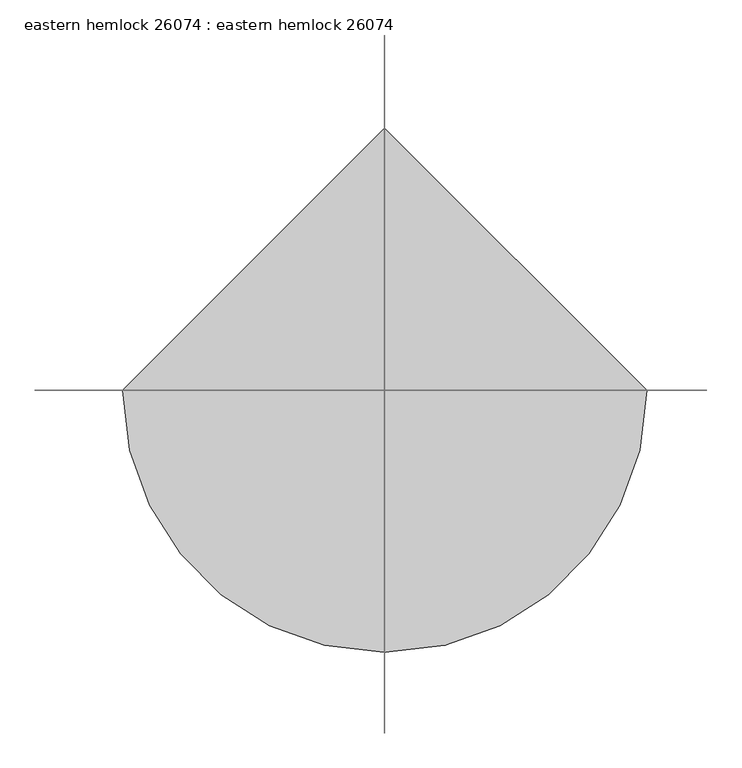
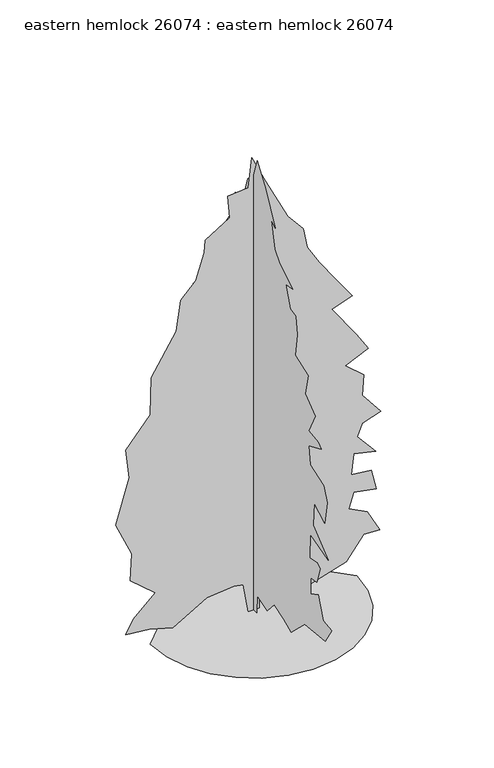
"""IFC4 building model written with IfcOpenShell, lengths in millimetres: proxy geometry, eastern hemlock 26074 : eastern hemlock 26074."""

import ifcopenshell
import ifcopenshell.guid

model = None  # the IFC model being written
_history = None  # IfcOwnerHistory: only IFC2X3 demands one
_inside = {}  # id of a spatial element -> (the spatial element, [elements in it])
_under = {}  # id of a project, library or spatial element -> (it, [spatial elements below it])
_declared = {}  # id of a project -> (the project, [libraries it declares])
_typed = {}  # id of a type object -> (the type object, [elements of that type])
_made_of = {}  # id of a material, layer set ... -> (it, [elements and type objects made of it])


def new_model(schema):
    """Start an empty IFC model of exactly this schema.

    Asked for "IFC4X3", IfcOpenShell would pick the latest addendum, in which some entities
    have other attributes; the version numbers below select the first issue.
    IFC2X3 requires an IfcOwnerHistory on every rooted entity: one is made here for all.
    """
    global model, _history
    if schema == "IFC4X3":
        model = ifcopenshell.file(schema_version=(4, 3, 0, 0))
    else:
        model = ifcopenshell.file(schema=schema)
    _inside.clear()
    _under.clear()
    _declared.clear()
    _typed.clear()
    _made_of.clear()
    _history = None
    if model.schema == "IFC2X3":
        org = make("IfcOrganization", Name="unknown")
        user = make(
            "IfcPersonAndOrganization",
            ThePerson=make("IfcPerson", FamilyName="unknown"),
            TheOrganization=org,
        )
        app = make(
            "IfcApplication",
            ApplicationDeveloper=org,
            Version="unknown",
            ApplicationFullName="unknown",
            ApplicationIdentifier="unknown",
        )
        _history = make(
            "IfcOwnerHistory",
            OwningUser=user,
            OwningApplication=app,
            ChangeAction="ADDED",
            CreationDate=0,
        )
    return model


def make(cls, **values):
    """One entity of the class cls with the attributes given. An attribute that is None is left unset."""
    return model.create_entity(
        cls, **{name: value for name, value in values.items() if value is not None}
    )


def rooted(cls, **values):
    """An entity with a GlobalId (a new one), such as an element, a storey or a relation."""
    return make(cls, GlobalId=ifcopenshell.guid.new(), OwnerHistory=_history, **values)


def si_unit(unit_type, name, prefix=None):
    """IfcSIUnit, for example si_unit("LENGTHUNIT", "METRE", prefix="MILLI")."""
    return make("IfcSIUnit", UnitType=unit_type, Prefix=prefix, Name=name)


def assignment(units):
    """IfcUnitAssignment: the units of a project."""
    return None if units is None else make("IfcUnitAssignment", Units=units)


def point(xyz):
    """IfcCartesianPoint."""
    return None if xyz is None else make("IfcCartesianPoint", Coordinates=xyz)


def direction(xyz):
    """IfcDirection."""
    return None if xyz is None else make("IfcDirection", DirectionRatios=xyz)


def frame(location, z_axis=None, x_axis=None):
    """IfcAxis2Placement3D, a coordinate frame: its origin and axes. An axis left out is left unset."""
    return make(
        "IfcAxis2Placement3D",
        Location=point(location),
        Axis=direction(z_axis),
        RefDirection=direction(x_axis),
    )


def origin():
    """The frame at (0, 0, 0) with its axes left unset."""
    return frame((0.0, 0.0, 0.0))


def place(relative_to, where):
    """IfcLocalPlacement: puts the frame where relative to a parent placement (None: the world)."""
    return make(
        "IfcLocalPlacement", PlacementRelTo=relative_to, RelativePlacement=where
    )


def context(
    kind, dimensions, precision=None, world=None, true_north=None, identifier=None
):
    """IfcGeometricRepresentationContext, for example the 3D "Model" context."""
    return make(
        "IfcGeometricRepresentationContext",
        ContextIdentifier=identifier,
        ContextType=kind,
        CoordinateSpaceDimension=dimensions,
        Precision=precision,
        WorldCoordinateSystem=world,
        TrueNorth=true_north,
    )


def project(units=None, contexts=None):
    """IfcProject with its units and contexts."""
    return rooted(
        "IfcProject",
        Name="project",
        RepresentationContexts=contexts,
        UnitsInContext=assignment(units),
    )


def spatial(cls, under=None, at=None, **own):
    """A site, building, storey or space (cls), placed at a placement, below another one or the project."""
    s = rooted(cls, ObjectPlacement=at, **own)
    if under is not None:
        _under.setdefault(under.id(), (under, []))[1].append(s)
    return s


def point_list(points):
    """IfcCartesianPointList2D or 3D."""
    cls = (
        "IfcCartesianPointList2D" if len(points[0]) == 2 else "IfcCartesianPointList3D"
    )
    return make(cls, CoordList=points)


def triangles(points, corners, closed=None, point_numbers=None):
    """IfcTriangulatedFaceSet: each triangle names its three corners, points numbered from 1."""
    return make(
        "IfcTriangulatedFaceSet",
        Coordinates=point_list(points),
        Closed=closed,
        CoordIndex=corners,
        PnIndex=point_numbers,
    )


def shape(context_of_items, identifier, shape_type, items):
    """IfcShapeRepresentation: the items that make up one representation, for example the "Body"."""
    return make(
        "IfcShapeRepresentation",
        ContextOfItems=context_of_items,
        RepresentationIdentifier=identifier,
        RepresentationType=shape_type,
        Items=items,
    )


def source(mapping_origin, context_of_items, identifier, shape_type, items):
    """IfcRepresentationMap: a shape defined once, which mapped items show again and again."""
    return make(
        "IfcRepresentationMap",
        MappingOrigin=mapping_origin,
        MappedRepresentation=shape(context_of_items, identifier, shape_type, items),
    )


def transform(
    local_origin,
    x_axis=None,
    y_axis=None,
    z_axis=None,
    scale=None,
    scale2=None,
    scale3=None,
    uniform=True,
):
    """IfcCartesianTransformationOperator3D, or its non-uniform kind. x_axis, y_axis, z_axis: its Axis1, 2, 3."""
    if uniform:
        return make(
            "IfcCartesianTransformationOperator3D",
            Axis1=direction(x_axis),
            Axis2=direction(y_axis),
            LocalOrigin=point(local_origin),
            Scale=scale,
            Axis3=direction(z_axis),
        )
    return make(
        "IfcCartesianTransformationOperator3DnonUniform",
        Axis1=direction(x_axis),
        Axis2=direction(y_axis),
        LocalOrigin=point(local_origin),
        Scale=scale,
        Axis3=direction(z_axis),
        Scale2=scale2,
        Scale3=scale3,
    )


def mapped(mapping_source, mapping_target):
    """IfcMappedItem: shows the shape of a source again, moved by a transform."""
    return make(
        "IfcMappedItem", MappingSource=mapping_source, MappingTarget=mapping_target
    )


def made_of(thing, what):
    """Note that an element or type object is made of a material, layer set ...; save() writes the relation."""
    if what is not None:
        _made_of.setdefault(what.id(), (what, []))[1].append(thing)
    return thing


def element(
    cls,
    number,
    at=None,
    inside=None,
    cuts=None,
    type_object=None,
    material=None,
    context=None,
    identifier="Body",
    shape_type=None,
    held_by="IfcProductDefinitionShape",
    body=None,
    shapes=None,
    **own,
):
    """One element of the class cls, such as IfcWall. Its Tag is "e" and its number.

    at: its placement. inside: the storey or other place that contains it. cuts: it is an
    opening in that element (IfcRelVoidsElement). A single representation is given by context,
    identifier, shape_type and body (its items); several are given by shapes. held_by: the class
    of the entity that holds the representations. save() writes the other relations.
    """
    e = rooted(cls, Tag="e%d" % number, ObjectPlacement=at, **own)
    if body is not None:
        shapes = [shape(context, identifier, shape_type, body)]
    if shapes is not None:
        e.Representation = make(held_by, Representations=shapes)
    if inside is not None:
        _inside.setdefault(inside.id(), (inside, []))[1].append(e)
    if cuts is not None:
        rooted(
            "IfcRelVoidsElement", RelatingBuildingElement=cuts, RelatedOpeningElement=e
        )
    if type_object is not None:
        _typed.setdefault(type_object.id(), (type_object, []))[1].append(e)
    return made_of(e, material)


def aggregate(whole, parts):
    """IfcRelAggregates: a whole, such as a stair, and the parts it consists of."""
    return rooted("IfcRelAggregates", RelatingObject=whole, RelatedObjects=parts)


def save(model, path):
    """Write the relations noted so far, then the file.

    IfcRelAggregates (storeys below a building ...), IfcRelContainedInSpatialStructure (elements
    in a storey), IfcRelDefinesByType, IfcRelAssociatesMaterial and IfcRelDeclares: one each for
    every whole, place, type object, material and project.
    """
    for whole, parts in _under.values():
        aggregate(whole, parts)
    for where, things in _inside.values():
        rooted(
            "IfcRelContainedInSpatialStructure",
            RelatedElements=things,
            RelatingStructure=where,
        )
    for kind, things in _typed.values():
        rooted("IfcRelDefinesByType", RelatedObjects=things, RelatingType=kind)
    for what, things in _made_of.values():
        rooted("IfcRelAssociatesMaterial", RelatedObjects=things, RelatingMaterial=what)
    for by, libraries in _declared.values():
        rooted("IfcRelDeclares", RelatingContext=by, RelatedDefinitions=libraries)
    model.write(path)


def eastern_hemlock_26074_eastern_hemlock_26074_32de6804(model_context):
    return source(origin(), model_context, "Body", "Tessellation", [
        triangles([(-1644.9506115, 0.0, 4.68e-05), (-1601.463295, -376.9127495, 4.68e-05), (-1477.6130058, -723.0483805, 4.68e-05), (-1283.3159992, -1028.488167, 4.68e-05), (-1028.488167, -1283.3159992, 4.68e-05), (-723.0483805, -1477.6130058, 4.68e-05), (-376.9127495, -1601.463295, 4.68e-05), (7.19e-05, -1644.9506115, 4.68e-05), (376.9127495, -1601.463295, 4.68e-05), (723.0483805, -1477.6130058, 4.68e-05), (1028.488167, -1283.3159992, 4.68e-05), (1283.3159992, -1028.488167, 4.68e-05), (1477.6130058, -723.0483805, 4.68e-05), (1601.463295, -376.9127495, 4.68e-05), (1644.9506115, 0.0001438, 4.68e-05), (-0.0002157, 1644.9506115, 4.68e-05), (-87.3035192, 3.8e-06, 7.6e-06), (-167.9385319, -2.15e-05, 483.8085503), (-315.7699336, -1.66e-05, 510.6868152), (-749.7665897, 5e-06, 466.2597304), (-1289.7701111, 4.76e-05, 146.9891475), (-1659.6825611, 5.73e-05, 255.3434076), (-2035.9781971, 7.14e-05, 295.6607868), (-1915.0259869, 5.33e-05, 510.6868152), (-1565.6086521, 1.88e-05, 833.2258123), (-1968.782444, 1.56e-05, 1182.6431471), (-1941.9042881, -1.2e-05, 1626.1367889), (-2197.2477139, -3.45e-05, 2190.5800976), (-1982.2215946, -8.72e-05, 2916.2981552), (-2035.9781971, -0.0001137, 3400.0912994), (-1646.2434105, -0.0001579, 3857.0369545), (-1632.8044052, -0.0001954, 4475.2216049), (-1229.6306133, -0.0002514, 5120.3049042), (-1162.4349329, -0.000284, 5617.5600174), (-920.5306578, -0.000309, 5859.4690887), (-786.1393696, -0.0003405, 6289.516095), (-772.700219, -0.0003531, 6491.1159988), (-384.3981211, -0.0003848, 6737.4195694), (-409.8438426, -0.0004058, 7109.3003586), (-87.3032649, -0.0004215, 7136.1737183), (-33.5482861, -0.0004527, 7619.9924423), (181.4795114, -0.0004349, 7163.0720764), (544.3366871, -0.0004075, 6437.344281), (786.2409622, -0.0004004, 6141.6884903), (853.4366426, -0.0003834, 5805.6973709), (1041.584388, -0.0003724, 5483.1688019), (1296.9278137, -0.0003619, 5120.3049042), (1565.7102448, -0.0003512, 4744.0040359), (1243.1712112, -0.0003299, 4623.0747894), (1632.9059978, -0.0003141, 4072.0476677), (1821.0536705, -0.0003039, 3762.9554878), (1458.1973305, -0.0002784, 3601.6909126), (1753.8580627, -0.0002761, 3346.3451614), (1726.9797615, -0.0002549, 3010.3796219), (2022.6406391, -0.0002454, 2634.0790443), (1726.9797615, -0.0002269, 2539.9975777), (1646.3450031, -0.0002113, 2338.4106091), (1942.0058807, -0.0002034, 1988.9932743), (1592.588546, -0.000193, 2069.6280327), (1552.2712395, -0.0001712, 1733.6498486), (1874.810273, -0.0001829, 1693.332542), (1955.4450314, -0.0001664, 1357.3517418), (1592.588546, -0.0001545, 1424.5473495), (1511.9537876, -0.0001358, 1169.2039965), (1807.6145199, -0.0001399, 1021.3736303), (2009.2014885, -0.0001263, 645.078067), (1753.8580627, -0.0001159, 658.5172176), (1471.6364811, -8.19e-05, 295.6607868), (907.1930998, -4.69e-05, 120.9521376), (463.7019287, -3.71e-05, 282.2216543), (87.4051209, -3.35e-05, 497.2477009), (87.4051209, -3.8e-06, 0.0), (4.1e-06, 91.4188294, 5.35e-05), (1.91e-05, 158.6147188, 403.1737919), (3.27e-05, 427.3977493, 456.9302854), (3.49e-05, 548.3498869, 349.4172984), (5.38e-05, 1032.1584372, 255.3434076), (6.46e-05, 1327.8192421, 174.7089036), (8.3e-05, 1730.993034, 188.1480178), (0.0001034, 2026.6537663, 430.0520568), (0.0001188, 2228.2407349, 645.078067), (0.0001026, 1865.3842495, 645.078067), (9.88e-05, 1583.1626678, 940.738872), (0.0001188, 1905.7017014, 1128.8891607), (0.0001321, 2120.7276752, 1249.8412983), (0.0001246, 1784.7494911, 1505.184724), (0.0001421, 1986.3364597, 1787.4063057), (0.0001369, 1798.1886417, 1894.9193653), (0.0001617, 2040.0929169, 2365.288765), (0.0001663, 2053.5345383, 2499.6799805), (0.0001615, 1892.2625507, 2580.3073265), (0.0001691, 1757.8713352, 3037.2526909), (0.0001843, 1865.3842495, 3386.6549103), (0.0001869, 1798.1886417, 3574.8178436), (0.0001943, 1730.993034, 3924.2197723), (0.0001899, 1435.3323017, 4219.9008522), (0.0002082, 1663.7974262, 4488.6835739), (0.0001969, 1260.6236343, 4717.1309669), (0.0002059, 1300.9409409, 4959.040329), (0.0002051, 1085.914967, 5254.6961197), (0.0002166, 1072.4758163, 5657.8697662), (0.0002054, 787.5744564, 5711.8955383), (0.0002156, 790.254162, 6047.6070236), (0.0002156, 494.5933934, 6491.1159988), (0.000223, 508.0325077, 6719.5631012), (0.000215, 293.0064793, 6773.334819), (0.0002206, 158.6142101, 7163.0720764), (0.0002182, -2.6552119, 7324.3366516), (0.0002228, -96.7291975, 7619.9924423), (0.0002019, -338.6349987, 7284.0013229), (0.0001757, -593.9783881, 6786.7717896), (0.0001825, -486.4654012, 6853.9543167), (0.0001655, -580.5392738, 6423.9073105), (0.0001557, -701.4914114, 6276.0797058), (0.0001321, -1077.7869747, 6047.6070236), (0.0001397, -889.6391567, 6020.7336639), (0.0001242, -1010.5912943, 5684.7681244), (0.0001164, -1158.4217331, 5644.4333771), (0.0001062, -1198.7391123, 5362.2139755), (9.69e-05, -1151.8202465, 4980.5791306), (7.72e-05, -1507.8390678, 4851.5221825), (7.04e-05, -1427.2043095, 4502.1199631), (5.19e-05, -1695.9867405, 4287.0839607), (4.93e-05, -1521.2780731, 3937.6564522), (3.67e-05, -1776.6214989, 3897.3467033), (3.11e-05, -1857.2562572, 3830.1638855), (4.17e-05, -1521.2780731, 3682.3359901), (3.11e-05, -1561.595525, 3386.6549103), (1.07e-05, -1937.8910156, 3265.7000839), (-3e-07, -2031.9649246, 3037.2526909), (-8.9e-06, -1964.7693169, 2647.5154335), (9e-06, -1667.4727833, 2801.7696808), (-1.3e-06, -1642.2276672, 2419.0453674), (-3e-05, -2058.8432259, 2083.0671833), (-3.7e-06, -1561.595525, 2217.4583988), (-1.51e-05, -1548.1563744, 1814.2846069), (-2.29e-05, -1749.743343, 1854.6020588), (-2.82e-05, -1830.3781013, 1800.8454563), (-3.24e-05, -1736.3041924, 1518.6238747), (-2.6e-05, -1575.0346756, 1491.7455734), (-3.4e-05, -1575.0346756, 1222.9629971), (-3.98e-05, -1776.6214989, 1330.4760567), (-5.68e-05, -1924.451865, 981.0562511), (-6.78e-05, -2152.9171349, 954.1779499), (-6.84e-05, -1978.2084675, 671.9562956), (-4.48e-05, -1413.7651588, 618.1998384), (-3.88e-05, -1037.4695955, 255.3434076), (-2.7e-05, -835.8826996, 349.4172984), (-1.25e-05, -567.1001595, 430.0520568), (-1.05e-05, -378.9523779, 215.0262827), (4.5e-06, -96.7289432, 295.6607868), (-3.7e-06, -83.2898198, 4.83e-05)], [[15, 16, 1], [14, 15, 1], [14, 1, 2], [13, 14, 2], [13, 2, 3], [13, 3, 4], [12, 13, 4], [11, 12, 4], [11, 4, 5], [11, 5, 6], [11, 6, 7], [11, 7, 8], [11, 8, 9], [11, 9, 10], [40, 41, 42], [57, 58, 59], [65, 66, 67], [61, 62, 63], [60, 61, 63], [22, 23, 24], [54, 55, 56], [47, 48, 49], [50, 51, 52], [22, 24, 25], [71, 72, 17], [71, 17, 18], [38, 39, 40], [21, 22, 25], [20, 21, 25], [64, 65, 67], [40, 42, 43], [38, 40, 43], [64, 67, 68], [64, 68, 69], [64, 69, 70], [64, 70, 71], [49, 50, 52], [36, 37, 38], [36, 38, 43], [35, 36, 43], [35, 43, 44], [35, 44, 45], [35, 45, 46], [34, 35, 46], [33, 34, 46], [33, 46, 47], [33, 47, 49], [32, 33, 49], [31, 32, 49], [31, 49, 52], [30, 31, 52], [29, 30, 52], [28, 29, 52], [27, 28, 52], [27, 52, 53], [27, 53, 54], [27, 54, 56], [27, 56, 57], [27, 57, 59], [27, 59, 60], [26, 27, 60], [25, 26, 60], [20, 25, 60], [19, 20, 60], [18, 19, 60], [71, 18, 60], [64, 71, 60], [64, 60, 63], [133, 134, 135], [110, 111, 112], [114, 115, 116], [80, 81, 82], [108, 109, 110], [125, 126, 127], [124, 125, 127], [143, 144, 145], [84, 85, 86], [130, 131, 132], [96, 97, 98], [86, 87, 88], [141, 142, 143], [143, 145, 146], [141, 143, 146], [79, 80, 82], [151, 152, 73], [151, 73, 74], [120, 121, 122], [129, 130, 132], [128, 129, 132], [104, 105, 106], [122, 123, 124], [83, 84, 86], [100, 101, 102], [137, 138, 139], [136, 137, 139], [136, 139, 140], [78, 79, 82], [78, 82, 83], [77, 78, 83], [89, 90, 91], [146, 147, 148], [117, 118, 119], [149, 150, 151], [108, 110, 112], [107, 108, 112], [106, 107, 112], [106, 112, 113], [104, 106, 113], [76, 77, 83], [75, 76, 83], [88, 89, 91], [103, 104, 113], [102, 103, 113], [102, 113, 114], [102, 114, 116], [102, 116, 117], [102, 117, 119], [102, 119, 120], [100, 102, 120], [99, 100, 120], [98, 99, 120], [98, 120, 122], [98, 122, 124], [96, 98, 124], [96, 124, 127], [96, 127, 128], [96, 128, 132], [95, 96, 132], [94, 95, 132], [93, 94, 132], [92, 93, 132], [92, 132, 133], [92, 133, 135], [91, 92, 135], [88, 91, 135], [88, 135, 136], [86, 88, 136], [83, 86, 136], [75, 83, 136], [74, 75, 136], [74, 136, 140], [151, 74, 140], [149, 151, 140], [149, 140, 141], [149, 141, 146], [149, 146, 148]], closed=False),
    ])


if __name__ == "__main__":
    model = new_model("IFC4")
    model_context = context("Model", 3, world=origin())
    ifc_project = project(units=[si_unit("LENGTHUNIT", "METRE", prefix="MILLI")], contexts=[model_context])
    site = spatial("IfcSite", under=ifc_project)
    building = spatial("IfcBuilding", under=site)
    placement = place(None, origin())
    eastern_hemlock_26074_eastern_hemlock_26074_shape = eastern_hemlock_26074_eastern_hemlock_26074_32de6804(model_context)
    element("IfcBuildingElementProxy", 1, Name="eastern hemlock 26074 : eastern hemlock 26074", ObjectType="eastern hemlock 26074 : eastern hemlock 26074", at=placement, inside=building, context=model_context, shape_type="MappedRepresentation", body=[
        mapped(eastern_hemlock_26074_eastern_hemlock_26074_shape, transform((0.0, 0.0, 0.0), x_axis=(1.0, 0.0, 0.0), y_axis=(0.0, 1.0, 0.0), z_axis=(0.0, 0.0, 1.0))),
    ])
    save(model, "model.ifc")

# Revit data of these elements
# Type "eastern hemlock 26074 : eastern hemlock 26074"
#   built-in parameter 1005195 = "RPC-16-G0VH-QEXX-MT47-S000-ST1L-LVER-AU"
#   Height = 0
